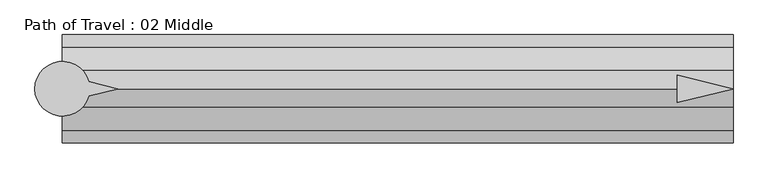
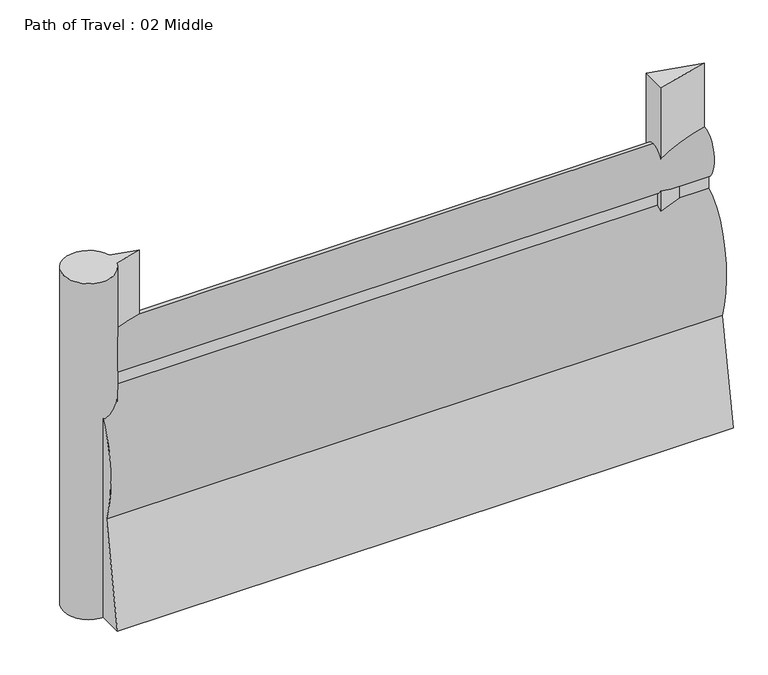
"""IFC4 building model written with IfcOpenShell, lengths in millimetres: proxy geometry, Path of Travel : 02 Middle."""

from ifc_helpers import new_model, si_unit, point, frame, frame_2d, origin, origin_with_axes, place, context, project, spatial, polyline, circle_curve, ellipse_curve, trimmed, segment, composite_curve, outline, extrude, source, transform, mapped, element, save
from ifc_brep_helpers import plane_surface, extruded_surface, advanced_brep


def path_of_travel_02_middle_a5fce673(model_context):
    return source(origin(), model_context, "Body", "SolidModel", [
        advanced_brep(
        [(227.5554837, 0.0, 1727.2), (227.5554837, 42.9018657, 1436.6534209), (227.5554837, 42.9018657, 1363.4763406), (227.5554837, 184.1186263, 643.4144547), (227.5554837, 297.5699544, 0.0), (227.5554837, 145.6574193, 0.0), (227.5554837, 0.0, 584.2), (227.5554837, -145.6574193, 0.0), (227.5554837, -297.5699544, 0.0), (227.5554837, -184.1186263, 643.4144547), (227.5554837, -42.9018657, 1363.4763406), (227.5554837, -42.9018657, 1436.6534209), (3916.3769655, 0.0, 1727.2), (3916.3769655, -42.9018657, 1436.6534209), (3916.3769655, -42.9018657, 1363.4763406), (3916.3769655, -184.1186263, 643.4144547), (3916.3769655, -297.5699544, 0.0), (3916.3769655, -145.6574193, 0.0), (3916.3769655, 0.0, 584.2), (3916.3769655, 145.6574193, 0.0), (3916.3769655, 297.5699544, 0.0), (3916.3769655, 184.1186263, 643.4144547), (3916.3769655, 42.9018657, 1363.4763406), (3916.3769655, 42.9018657, 1436.6534209)],
        [
            (0, 1, ellipse_curve(frame((227.5554837, 0.0, 1574.8), z_axis=(-1.0, 0.0, 0.0), x_axis=(0.0, 0.0, 1.0)), 152.4, 101.6)),
            (1, 2),
            (2, 3, ellipse_curve(frame((227.5554837, 0.0, 914.4), z_axis=(-1.0, 0.0, 0.0), x_axis=(0.0, 0.0, -1.0)), 457.2, 228.6)),
            (3, 4),
            (4, 5),
            (5, 6),
            (6, 7),
            (7, 8),
            (8, 9),
            (9, 10, ellipse_curve(frame((227.5554837, 0.0, 914.4), z_axis=(-1.0, 0.0, 0.0), x_axis=(0.0, 0.0, -1.0)), 457.2, 228.6)),
            (10, 11),
            (11, 0, ellipse_curve(frame((227.5554837, 0.0, 1574.8), z_axis=(-1.0, 0.0, 0.0), x_axis=(0.0, 0.0, 1.0)), 152.4, 101.6)),
            (12, 13, ellipse_curve(frame((3916.3769655, 0.0, 1574.8), z_axis=(1.0, 0.0, 0.0), x_axis=(0.0, 0.0, 1.0)), 152.4, 101.6)),
            (13, 14),
            (14, 15, ellipse_curve(frame((3916.3769655, 0.0, 914.4), z_axis=(1.0, 0.0, 0.0), x_axis=(0.0, 0.0, -1.0)), 457.2, 228.6)),
            (15, 16),
            (16, 17),
            (17, 18),
            (18, 19),
            (19, 20),
            (20, 21),
            (21, 22, ellipse_curve(frame((3916.3769655, 0.0, 914.4), z_axis=(1.0, 0.0, 0.0), x_axis=(0.0, 0.0, -1.0)), 457.2, 228.6)),
            (22, 23),
            (23, 12, ellipse_curve(frame((3916.3769655, 0.0, 1574.8), z_axis=(1.0, 0.0, 0.0), x_axis=(0.0, 0.0, 1.0)), 152.4, 101.6)),
            (0, 12),
            (23, 1),
            (22, 2),
            (21, 3),
            (20, 4),
            (19, 5),
            (18, 6),
            (17, 7),
            (16, 8),
            (15, 9),
            (14, 10),
            (13, 11),
        ],
        [
            plane_surface(frame((227.5554837, 0.0, 0.0), z_axis=(-1.0, 0.0, 0.0), x_axis=(0.0, 0.0, 1.0))),
            plane_surface(frame((3916.3769655, 0.0, 0.0), z_axis=(1.0, 0.0, 0.0), x_axis=(0.0, 0.0, 1.0))),
            extruded_surface(trimmed(ellipse_curve(frame((3916.3769655, 0.0, 1574.8), z_axis=(-1.0, 0.0, 0.0), x_axis=(0.0, 0.0, 1.0)), 152.4, 101.6), [point((3916.3769655, 0.0, 1727.2))], [point((3916.3769655, 42.9018657, 1436.6534209))], True, "CARTESIAN"), (-3688.8214818, 0.0, 0.0), 3688.8214818),
            plane_surface(frame((227.5554837, 42.9018657, 1436.6534209), z_axis=(0.0, 1.0, 0.0), x_axis=(1.0, 0.0, 0.0))),
            extruded_surface(trimmed(ellipse_curve(frame((3916.3769655, 0.0, 914.4), z_axis=(-1.0, 0.0, 0.0), x_axis=(0.0, 0.0, -1.0)), 457.2, 228.6), [point((3916.3769655, 42.9018657, 1363.4763406))], [point((3916.3769655, 184.1186263, 643.4144547))], True, "CARTESIAN"), (-3688.8214818, 0.0, 0.0), 3688.8214818),
            plane_surface(frame((227.5554837, 184.1186263, 643.4144547), z_axis=(0.0, 0.9848077530122078, 0.1736481776669322), x_axis=(1.0, 0.0, 0.0))),
            plane_surface(frame((227.5554837, 297.5699544, 0.0), z_axis=(0.0, 0.0, -1.0), x_axis=(1.0, 0.0, 0.0))),
            plane_surface(frame((227.5554837, 145.6574193, 0.0), z_axis=(0.0, -0.9702957262760199, -0.2419218955995739), x_axis=(1.0, 0.0, 0.0))),
            plane_surface(frame((227.5554837, 0.0, 584.2), z_axis=(0.0, 0.9702957262759961, -0.24192189559966923), x_axis=(1.0, 0.0, 0.0))),
            plane_surface(frame((227.5554837, -145.6574193, 0.0), z_axis=(0.0, 0.0, -1.0), x_axis=(1.0, 0.0, 0.0))),
            plane_surface(frame((227.5554837, -297.5699544, 0.0), z_axis=(0.0, -0.984807753012208, 0.17364817766693066), x_axis=(1.0, 0.0, 0.0))),
            extruded_surface(trimmed(ellipse_curve(frame((3916.3769655, 0.0, 914.4), z_axis=(-1.0, 0.0, 0.0), x_axis=(0.0, 0.0, -1.0)), 457.2, 228.6), [point((3916.3769655, -184.1186263, 643.4144547))], [point((3916.3769655, -42.9018657, 1363.4763406))], True, "CARTESIAN"), (-3688.8214818, 0.0, 0.0), 3688.8214818),
            plane_surface(frame((227.5554837, -42.9018657, 1363.4763406), z_axis=(0.0, -1.0, 0.0), x_axis=(1.0, 0.0, 0.0))),
            extruded_surface(trimmed(ellipse_curve(frame((3916.3769655, 0.0, 1574.8), z_axis=(-1.0, 0.0, 0.0), x_axis=(0.0, 0.0, 1.0)), 152.4, 101.6), [point((3916.3769655, -42.9018657, 1436.6534209))], [point((3916.3769655, 0.0, 1727.2))], True, "CARTESIAN"), (-3688.8214818, 0.0, 0.0), 3688.8214818),
        ],
        [
            (0, [[1, 2, 3, 4, 5, 6, 7, 8, 9, 10, 11, 12]]),
            (1, [[13, 14, 15, 16, 17, 18, 19, 20, 21, 22, 23, 24]]),
            (2, [[-1, 25, -24, 26]]),
            (3, [[-2, -26, -23, 27]]),
            (4, [[-3, -27, -22, 28]]),
            (5, [[-4, -28, -21, 29]]),
            (6, [[-5, -29, -20, 30]]),
            (7, [[-6, -30, -19, 31]]),
            (8, [[-7, -31, -18, 32]]),
            (9, [[-8, -32, -17, 33]]),
            (10, [[-9, -33, -16, 34]]),
            (11, [[-10, -34, -15, 35]]),
            (12, [[-11, -35, -14, 36]]),
            (13, [[-12, -36, -13, -25]]),
        ],
    ),
        extrude(outline(polyline([(3610.371819, 76.2006338), (3916.3769655, 0.0), (3610.371819, -76.2006338), (3610.371819, 76.2006338)])), origin_with_axes(), (0.0, 0.0, 1.0), 2129.5973753),
        extrude(outline(composite_curve([segment(polyline([(372.7837828, 39.4440225), (531.182385, 0.0), (372.7837828, -39.4440225)]), True, "CONTINUOUS"), segment(trimmed(circle_curve(frame_2d((227.2200886, 0.0)), 150.8131956), [point((372.7837828, -39.4440225))], [point((372.7837828, 39.4440225))], False, "CARTESIAN"), True, "CONTINUOUS")], self_intersect=False)), origin_with_axes(), (0.0, 0.0, 1.0), 2129.5973753),
    ])


if __name__ == "__main__":
    model = new_model("IFC4")
    model_context = context("Model", 3, world=origin())
    ifc_project = project(units=[si_unit("LENGTHUNIT", "METRE", prefix="MILLI")], contexts=[model_context])
    site = spatial("IfcSite", under=ifc_project)
    building = spatial("IfcBuilding", under=site)
    placement = place(None, origin())
    path_of_travel_02_middle_shape = path_of_travel_02_middle_a5fce673(model_context)
    element("IfcBuildingElementProxy", 1, Name="Path of Travel : 02 Middle", ObjectType="Path of Travel : 02 Middle", at=placement, inside=building, context=model_context, shape_type="MappedRepresentation", body=[
        mapped(path_of_travel_02_middle_shape, transform((0.0, 0.0, 0.0), x_axis=(1.0, 0.0, 0.0), y_axis=(0.0, 1.0, 0.0), z_axis=(0.0, 0.0, 1.0))),
    ])
    save(model, "model.ifc")

# Revit data of these elements
# Type "Path of Travel : 02 Middle"
#   Path of Egress [instance default] = 4' - 0"
#   built-in parameter 1001306 [instance default] = 4 (stored number, unit not read)
#   Dot at Start = no
#   Arrow in Middle = yes
#   Arrow at End = no
#   Egress Path = none
# Element 1 (IfcBuildingElementProxy, "Path of Travel : 02 Middle")
#   Path of Egress = 12' - 1.22919"
#   built-in parameter 1001306 = 12.1024 (stored number, unit not read)
